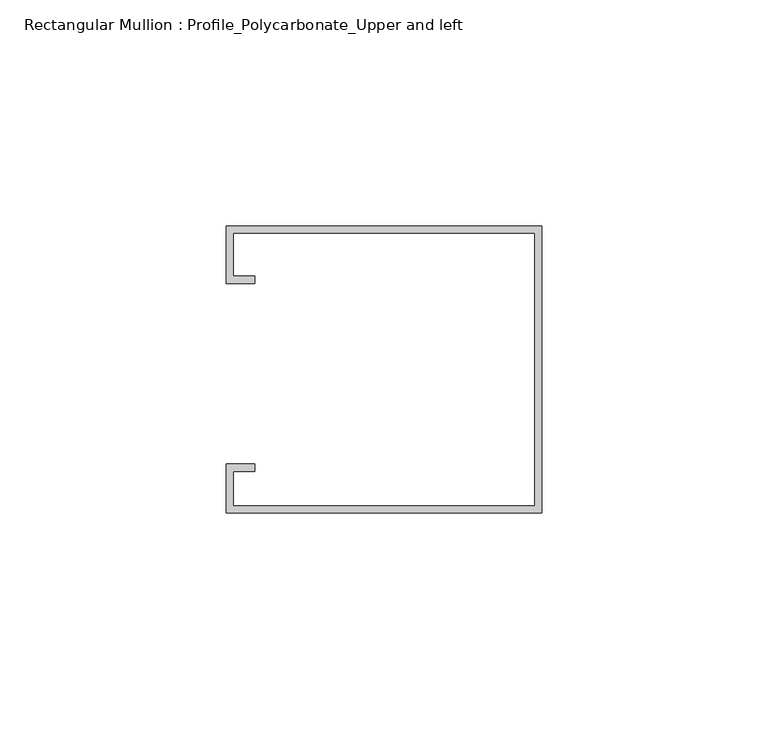
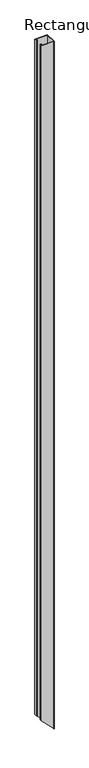
"""IFC4 building model written with IfcOpenShell, lengths in millimetres: member geometry, Rectangular Mullion : Profile_Polycarbonate_Upper and left."""

from ifc_helpers import new_model, si_unit, origin, place, context, project, spatial, faceted_brep, source, transform, mapped, element, save


def rectangular_mullion_profile_polycarbonate_upper_and_left_6bbbb23a(model_context):
    return source(origin(), model_context, "Body", "Brep", [
        faceted_brep([(0.0, 32.7, 0.0), (-69.85, 32.7, 0.0), (-69.85, 20.0, 0.0), (-63.5, 20.0, 0.0), (-63.5, 21.5875, 0.0), (-68.2625, 21.5875, 0.0), (-68.2625, 31.1125, 0.0), (-1.5875, 31.1125, 0.0), (-1.5875, -29.2125, 0.0), (-68.2625, -29.2125, 0.0), (-68.2625, -21.5875, 0.0), (-63.5, -21.5875, 0.0), (-63.5, -20.0, 0.0), (-69.85, -20.0, 0.0), (-69.85, -30.8, 0.0), (0.0, -30.8, 0.0), (0.0, 32.7, -4050.9028356), (-69.85, 32.7, -3978.0818115), (-69.85, 20.0, -3978.0818115), (-63.5, 20.0, -3984.7019046), (-63.5, 21.5875, -3984.7019046), (-68.2625, 21.5875, -3979.7368348), (-68.2625, 31.1125, -3979.7368348), (-1.5875, 31.1125, -4049.2478123), (-1.5875, -29.2125, -4049.2478123), (-68.2625, -29.2125, -3979.7368348), (-68.2625, -21.5875, -3979.7368348), (-63.5, -21.5875, -3984.7019046), (-63.5, -20.0, -3984.7019046), (-69.85, -20.0, -3978.0818115), (-69.85, -30.8, -3978.0818115), (0.0, -30.8, -4050.9028356)], [[[0, 1, 2, 3, 4, 5, 6, 7, 8, 9, 10, 11, 12, 13, 14, 15]], [[1, 0, 16, 17]], [[2, 1, 17, 18]], [[3, 2, 18, 19]], [[4, 3, 19, 20]], [[5, 4, 20, 21]], [[6, 5, 21, 22]], [[7, 6, 22, 23]], [[8, 7, 23, 24]], [[9, 8, 24, 25]], [[10, 9, 25, 26]], [[11, 10, 26, 27]], [[12, 11, 27, 28]], [[13, 12, 28, 29]], [[14, 13, 29, 30]], [[15, 14, 30, 31]], [[0, 15, 31, 16]], [[16, 31, 30, 29, 28, 27, 26, 25, 24, 23, 22, 21, 20, 19, 18, 17]]]),
    ])


if __name__ == "__main__":
    model = new_model("IFC4")
    model_context = context("Model", 3, world=origin())
    ifc_project = project(units=[si_unit("LENGTHUNIT", "METRE", prefix="MILLI")], contexts=[model_context])
    site = spatial("IfcSite", under=ifc_project)
    building = spatial("IfcBuilding", under=site)
    placement = place(None, origin())
    rectangular_mullion_profile_polycarbonate_upper_and_left_shape = rectangular_mullion_profile_polycarbonate_upper_and_left_6bbbb23a(model_context)
    element("IfcMember", 1, ObjectType="Rectangular Mullion : Profile_Polycarbonate_Upper and left", at=placement, inside=building, context=model_context, shape_type="MappedRepresentation", body=[
        mapped(rectangular_mullion_profile_polycarbonate_upper_and_left_shape, transform((0.0, 0.0, 0.0), x_axis=(1.0, 0.0, 0.0), y_axis=(0.0, 1.0, 0.0), z_axis=(0.0, 0.0, 1.0))),
    ])
    save(model, "model.ifc")

# Revit data of these elements
# Type "Rectangular Mullion : Profile_Polycarbonate_Upper and left"
#   built-in parameter 1007322 = 0.208333 (stored number, unit not read)
#   built-in parameter 1007321 = 0.00520833 (stored number, unit not read)
#   built-in parameter 1007320 = 0 (stored number, unit not read)
